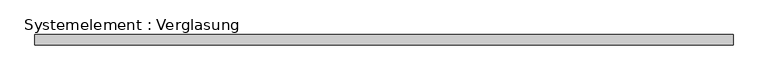
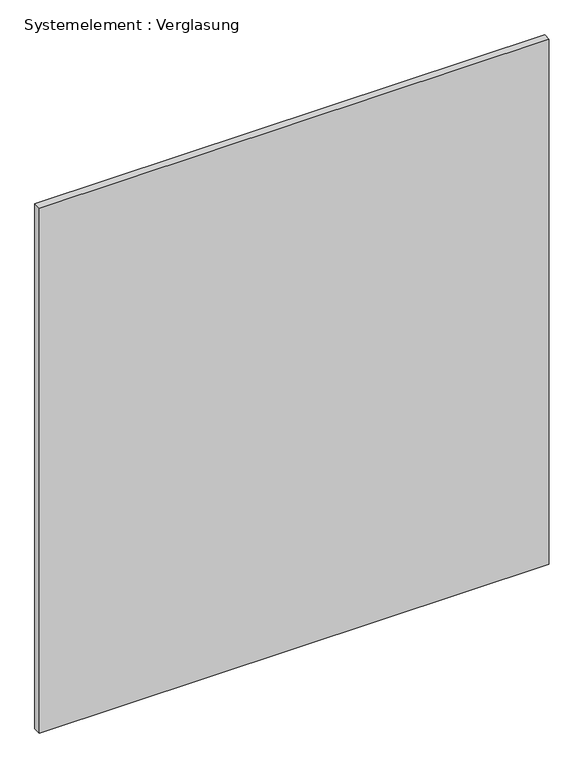
"""IFC4 building model written with IfcOpenShell, lengths in millimetres: plate geometry, Systemelement : Verglasung."""

from ifc_helpers import new_model, si_unit, origin, origin_with_axes, place, context, project, spatial, polyline, outline, extrude, source, transform, mapped, element, save


def systemelement_verglasung_c088afcf(model_context):
    return source(origin(), model_context, "Body", "SweptSolid", [
        extrude(outline(polyline([(1025.0000002, -15.0), (-1025.0000002, -15.0), (-1025.0000002, 15.0), (1025.0000002, 15.0), (1025.0000002, -15.0)])), origin_with_axes(), (0.0, 0.0, 1.0), 2230.0),
    ])


if __name__ == "__main__":
    model = new_model("IFC4")
    model_context = context("Model", 3, world=origin())
    ifc_project = project(units=[si_unit("LENGTHUNIT", "METRE", prefix="MILLI")], contexts=[model_context])
    site = spatial("IfcSite", under=ifc_project)
    building = spatial("IfcBuilding", under=site)
    placement = place(None, origin())
    systemelement_verglasung_shape = systemelement_verglasung_c088afcf(model_context)
    element("IfcPlate", 1, ObjectType="Systemelement : Verglasung", at=placement, inside=building, context=model_context, shape_type="MappedRepresentation", body=[
        mapped(systemelement_verglasung_shape, transform((0.0, 0.0, 0.0), x_axis=(1.0, 0.0, 0.0), y_axis=(0.0, 1.0, 0.0), z_axis=(0.0, 0.0, 1.0))),
    ])
    save(model, "model.ifc")

# Revit data of these elements
# Type "Systemelement : Verglasung"
#   Construction Type Id = "GSP4R"
#   Analytic Construction = "1/8 Zoll Pilkington-Verglasung einfach"
#   Visual Light Transmittance = 0.9
#   Solar Heat Gain Coefficient = 0.86
#   Heat Transfer Coefficient (U) = 6.7069 W/(m²·K)
# Element 1 (IfcPlate, "Systemelement : Verglasung")
#   Materials on its faces: "Glas"
# Materials
#   "Glas": class "Glas", colour RGB 0 0 255, transparency 0.75, Comments = "Render-Darstellung nicht aktualisiert ", Cost = 0
